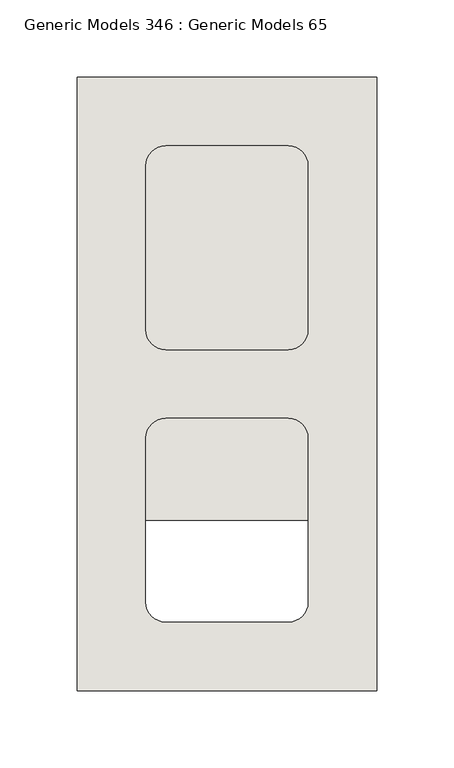
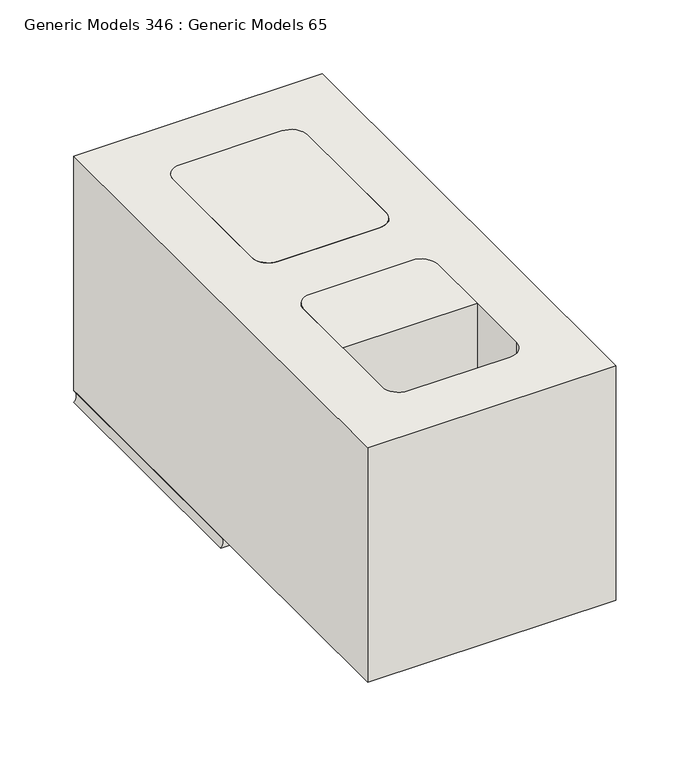
"""IFC4 building model written with IfcOpenShell, lengths in millimetres: wall geometry, Generic Models 346 : Generic Models 65."""

from ifc_helpers import new_model, si_unit, point, frame, frame_2d, origin, place, context, project, spatial, polyline, circle_curve, trimmed, segment, composite_curve, outline, extrude, source, transform, mapped, element, save
from ifc_brep_helpers import plane_surface, revolved_surface, advanced_brep


def generic_models_346_generic_models_65_9e6e97e0(model_context):
    return source(origin(), model_context, "Body", "SolidModel", [
        advanced_brep(
        [(430198.2125, 503.2375, 619.125), (430004.5375, 503.2375, 619.125), (430004.5375, 503.2375, 609.6), (430198.2125, 503.2375, 609.6), (430198.2125, 701.675, 619.125), (430198.2125, 701.675, 609.6), (430004.5375, 701.675, 609.6), (430004.5375, 701.675, 619.125), (430153.7625, 538.1625, 619.125), (430141.0625, 525.4625, 619.125), (430061.6875, 525.4625, 619.125), (430048.9875, 538.1625, 619.125), (430048.9875, 644.525, 619.125), (430061.6875, 657.225, 619.125), (430141.0625, 657.225, 619.125), (430153.7625, 644.525, 619.125), (430141.0625, 525.4625, 609.6), (430153.7625, 538.1625, 609.6), (430061.6875, 525.4625, 609.6), (430048.9875, 538.1625, 609.6), (430048.9875, 644.525, 609.6), (430061.6875, 657.225, 609.6), (430141.0625, 657.225, 609.6), (430153.7625, 644.525, 609.6)],
        [
            (0, 1),
            (1, 2, circle_curve(frame((429999.6545028, 503.2375, 614.3625), z_axis=(0.0, 1.0, 0.0), x_axis=(1.0, 0.0, 0.0)), 6.8209287)),
            (2, 3),
            (3, 0, circle_curve(frame((430203.0954972, 503.2375, 614.3625), z_axis=(0.0, 1.0, 0.0), x_axis=(-1.0, 0.0, 0.0)), 6.8209287)),
            (4, 5, circle_curve(frame((430203.0954972, 701.675, 614.3625), z_axis=(0.0, -1.0, 0.0), x_axis=(-1.0, 0.0, 0.0)), 6.8209287)),
            (5, 6),
            (6, 7, circle_curve(frame((429999.6545028, 701.675, 614.3625), z_axis=(0.0, -1.0, 0.0), x_axis=(1.0, 0.0, 0.0)), 6.8209287)),
            (7, 4),
            (0, 4),
            (7, 1),
            (8, 9, circle_curve(frame((430141.0625, 538.1625, 619.125), z_axis=(0.0, 0.0, -1.0), x_axis=(-1.0, 0.0, 0.0)), 12.7)),
            (9, 10),
            (10, 11, circle_curve(frame((430061.6875, 538.1625, 619.125), z_axis=(0.0, 0.0, -1.0), x_axis=(-1.0, 0.0, 0.0)), 12.7)),
            (11, 12),
            (12, 13, circle_curve(frame((430061.6875, 644.525, 619.125), z_axis=(0.0, 0.0, -1.0), x_axis=(-1.0, 0.0, 0.0)), 12.7)),
            (13, 14),
            (14, 15, circle_curve(frame((430141.0625, 644.525, 619.125), z_axis=(0.0, 0.0, -1.0), x_axis=(-1.0, 0.0, 0.0)), 12.7)),
            (15, 8),
            (16, 9),
            (8, 17),
            (17, 16, circle_curve(frame((430141.0625, 538.1625, 609.6), z_axis=(0.0, 0.0, -1.0), x_axis=(-1.0, 0.0, 0.0)), 12.7)),
            (16, 18),
            (18, 10),
            (18, 19, circle_curve(frame((430061.6875, 538.1625, 609.6), z_axis=(0.0, 0.0, -1.0), x_axis=(-1.0, 0.0, 0.0)), 12.7)),
            (19, 11),
            (19, 20),
            (20, 12),
            (20, 21, circle_curve(frame((430061.6875, 644.525, 609.6), z_axis=(0.0, 0.0, -1.0), x_axis=(-1.0, 0.0, 0.0)), 12.7)),
            (21, 13),
            (21, 22),
            (22, 14),
            (22, 23, circle_curve(frame((430141.0625, 644.525, 609.6), z_axis=(0.0, 0.0, -1.0), x_axis=(-1.0, 0.0, 0.0)), 12.7)),
            (23, 15),
            (23, 17),
            (6, 2),
            (5, 3),
        ],
        [
            plane_surface(frame((430101.375, 503.2375, 619.521875), z_axis=(0.0, -1.0, 0.0), x_axis=(0.0, 0.0, 1.0))),
            plane_surface(frame((430101.375, 701.675, 619.521875), z_axis=(0.0, 1.0, 0.0), x_axis=(0.0, 0.0, 1.0))),
            plane_surface(frame((430198.2125, 503.2375, 619.125), z_axis=(0.0, 0.0, 1.0), x_axis=(0.0, 1.0, 0.0))),
            revolved_surface(polyline([(430128.3625, 538.1625, 619.125), (430128.3625, 538.1625, 609.6)]), (430141.0625, 538.1625, 803.275), (0.0, 0.0, 1.0)),
            plane_surface(frame((430061.6875, 525.4625, 803.275), z_axis=(0.0, 1.0, 0.0), x_axis=(0.0, 0.0, -1.0))),
            revolved_surface(polyline([(430048.9875, 538.1625, 619.125), (430048.9875, 538.1625, 609.6)]), (430061.6875, 538.1625, 803.275), (0.0, 0.0, 1.0)),
            plane_surface(frame((430048.9875, 644.525, 803.275), z_axis=(1.0, 0.0, 0.0), x_axis=(0.0, 0.0, -1.0))),
            revolved_surface(polyline([(430048.9875, 644.525, 619.125), (430048.9875, 644.525, 609.6)]), (430061.6875, 644.525, 803.275), (0.0, 0.0, 1.0)),
            plane_surface(frame((430141.0625, 657.225, 803.275), z_axis=(0.0, -1.0, 0.0), x_axis=(0.0, 0.0, -1.0))),
            revolved_surface(polyline([(430128.3625, 644.525, 619.125), (430128.3625, 644.525, 609.6)]), (430141.0625, 644.525, 803.275), (0.0, 0.0, 1.0)),
            plane_surface(frame((430153.7625, 538.1625, 803.275), z_axis=(-1.0, 0.0, 0.0), x_axis=(0.0, 0.0, -1.0))),
            revolved_surface(polyline([(430006.4754315, 701.675, 614.3625), (430006.4754315, 503.2375, 614.3625)]), (429999.6545028, 503.2375, 614.3625), (0.0, 1.0, 0.0)),
            plane_surface(frame((430004.5375, 503.2375, 609.6), z_axis=(0.0, 0.0, -1.0), x_axis=(0.0, 1.0, 0.0))),
            revolved_surface(polyline([(430196.2745685, 701.675, 614.3625), (430196.2745685, 503.2375, 614.3625)]), (430203.0954972, 503.2375, 614.3625), (0.0, 1.0, 0.0)),
        ],
        [
            (0, [[1, 2, 3, 4]]),
            (1, [[5, 6, 7, 8]]),
            (2, [[-1, 9, -8, 10], [11, 12, 13, 14, 15, 16, 17, 18]]),
            (3, [[19, -11, 20, 21]]),
            (4, [[-19, 22, 23, -12]]),
            (5, [[-23, 24, 25, -13]]),
            (6, [[-25, 26, 27, -14]]),
            (7, [[-27, 28, 29, -15]]),
            (8, [[-29, 30, 31, -16]]),
            (9, [[-31, 32, 33, -17]]),
            (10, [[-33, 34, -20, -18]]),
            (11, [[-2, -10, -7, 35]]),
            (12, [[-3, -35, -6, 36], [-21, -34, -32, -30, -28, -26, -24, -22]]),
            (13, [[-4, -36, -5, -9]]),
        ],
    ),
        extrude(outline(composite_curve([segment(trimmed(circle_curve(frame_2d((430141.0625, 538.1625)), 12.7), [point((430153.7625, 538.1625))], [point((430141.0625, 525.4625))], False, "CARTESIAN"), True, "CONTINUOUS"), segment(polyline([(430141.0625, 525.4625), (430061.6875, 525.4625)]), True, "CONTINUOUS"), segment(trimmed(circle_curve(frame_2d((430061.6875, 538.1625)), 12.7), [point((430061.6875, 525.4625))], [point((430048.9875, 538.1625))], False, "CARTESIAN"), True, "CONTINUOUS"), segment(polyline([(430048.9875, 538.1625), (430048.9875, 644.525)]), True, "CONTINUOUS"), segment(trimmed(circle_curve(frame_2d((430061.6875, 644.525)), 12.7), [point((430048.9875, 644.525))], [point((430061.6875, 657.225))], False, "CARTESIAN"), True, "CONTINUOUS"), segment(polyline([(430061.6875, 657.225), (430141.0625, 657.225)]), True, "CONTINUOUS"), segment(trimmed(circle_curve(frame_2d((430141.0625, 644.525)), 12.7), [point((430141.0625, 657.225))], [point((430153.7625, 644.525))], False, "CARTESIAN"), True, "CONTINUOUS"), segment(polyline([(430153.7625, 644.525), (430153.7625, 538.1625)]), True, "CONTINUOUS")], self_intersect=False)), frame((0.0, 0.0, 609.6), z_axis=(0.0, 0.0, 1.0), x_axis=(1.0, 0.0, 0.0)), (0.0, 0.0, 1.0), 203.2),
        extrude(outline(composite_curve([segment(trimmed(circle_curve(frame_2d((430061.6875, 468.3125)), 12.7), [point((430048.9875, 468.3125))], [point((430061.6875, 481.0125))], False, "CARTESIAN"), True, "CONTINUOUS"), segment(polyline([(430061.6875, 481.0125), (430141.0625, 481.0125)]), True, "CONTINUOUS"), segment(trimmed(circle_curve(frame_2d((430141.0625, 468.3125)), 12.7), [point((430141.0625, 481.0125))], [point((430153.7625, 468.3125))], False, "CARTESIAN"), True, "CONTINUOUS"), segment(polyline([(430153.7625, 468.3125), (430153.7625, 415.13125), (430048.9875, 415.13125), (430048.9875, 468.3125)]), True, "CONTINUOUS")], self_intersect=False)), frame((0.0, 0.0, 609.6), z_axis=(0.0, 0.0, 1.0), x_axis=(1.0, 0.0, 0.0)), (0.0, 0.0, 1.0), 203.2),
        extrude(outline(polyline([(430198.2125, 304.8), (430004.5375, 304.8), (430004.5375, 701.675), (430198.2125, 701.675), (430198.2125, 304.8)]), holes=[composite_curve([segment(polyline([(430153.7625, 538.1625), (430153.7625, 644.525)]), True, "CONTINUOUS"), segment(trimmed(circle_curve(frame_2d((430141.0625, 644.525)), 12.7), [point((430153.7625, 644.525))], [point((430141.0625, 657.225))], True, "CARTESIAN"), True, "CONTINUOUS"), segment(polyline([(430141.0625, 657.225), (430061.6875, 657.225)]), True, "CONTINUOUS"), segment(trimmed(circle_curve(frame_2d((430061.6875, 644.525)), 12.7), [point((430061.6875, 657.225))], [point((430048.9875, 644.525))], True, "CARTESIAN"), True, "CONTINUOUS"), segment(polyline([(430048.9875, 644.525), (430048.9875, 538.1625)]), True, "CONTINUOUS"), segment(trimmed(circle_curve(frame_2d((430061.6875, 538.1625)), 12.7), [point((430048.9875, 538.1625))], [point((430061.6875, 525.4625))], True, "CARTESIAN"), True, "CONTINUOUS"), segment(polyline([(430061.6875, 525.4625), (430141.0625, 525.4625)]), True, "CONTINUOUS"), segment(trimmed(circle_curve(frame_2d((430141.0625, 538.1625)), 12.7), [point((430141.0625, 525.4625))], [point((430153.7625, 538.1625))], True, "CARTESIAN"), True, "CONTINUOUS")], self_intersect=False), composite_curve([segment(polyline([(430048.9875, 468.3125), (430048.9875, 361.95)]), True, "CONTINUOUS"), segment(trimmed(circle_curve(frame_2d((430061.6875, 361.95)), 12.7), [point((430048.9875, 361.95))], [point((430061.6875, 349.25))], True, "CARTESIAN"), True, "CONTINUOUS"), segment(polyline([(430061.6875, 349.25), (430141.0625, 349.25)]), True, "CONTINUOUS"), segment(trimmed(circle_curve(frame_2d((430141.0625, 361.95)), 12.7), [point((430141.0625, 349.25))], [point((430153.7625, 361.95))], True, "CARTESIAN"), True, "CONTINUOUS"), segment(polyline([(430153.7625, 361.95), (430153.7625, 468.3125)]), True, "CONTINUOUS"), segment(trimmed(circle_curve(frame_2d((430141.0625, 468.3125)), 12.7), [point((430153.7625, 468.3125))], [point((430141.0625, 481.0125))], True, "CARTESIAN"), True, "CONTINUOUS"), segment(polyline([(430141.0625, 481.0125), (430061.6875, 481.0125)]), True, "CONTINUOUS"), segment(trimmed(circle_curve(frame_2d((430061.6875, 468.3125)), 12.7), [point((430061.6875, 481.0125))], [point((430048.9875, 468.3125))], True, "CARTESIAN"), True, "CONTINUOUS")], self_intersect=False)]), frame((0.0, 0.0, 619.125), z_axis=(0.0, 0.0, 1.0), x_axis=(1.0, 0.0, 0.0)), (0.0, 0.0, 1.0), 193.675),
    ])


if __name__ == "__main__":
    model = new_model("IFC4")
    model_context = context("Model", 3, world=origin())
    ifc_project = project(units=[si_unit("LENGTHUNIT", "METRE", prefix="MILLI")], contexts=[model_context])
    site = spatial("IfcSite", under=ifc_project)
    building = spatial("IfcBuilding", under=site)
    placement = place(None, origin())
    generic_models_346_generic_models_65_shape = generic_models_346_generic_models_65_9e6e97e0(model_context)
    element("IfcWall", 1, ObjectType="Generic Models 346 : Generic Models 65", at=placement, inside=building, context=model_context, shape_type="MappedRepresentation", body=[
        mapped(generic_models_346_generic_models_65_shape, transform((0.0, 0.0, 0.0), x_axis=(1.0, 0.0, 0.0), y_axis=(0.0, 1.0, 0.0), z_axis=(0.0, 0.0, 1.0))),
    ])
    save(model, "model.ifc")

# Revit data of these elements
# Element 1 (IfcWall, "Generic Models 346 : Generic Models 65")
#   Materials on its faces: "CMU (SEE 'WALL TAG' FOR SIZE)", "FILL CORE IF APPLICABLE - SEE STRUCTURAL DWGS FOR DETAILS", "MORTAR JOINT"
# Materials
#   "CMU (SEE 'WALL TAG' FOR SIZE)": class "Masonry", colour RGB 203 203 199, transparency 0, Description = "Concrete masonry units", Cost = 0
#   "FILL CORE IF APPLICABLE - SEE STRUCTURAL DWGS FOR DETAILS": class "Generic", colour RGB 170 170 170, transparency 0, Cost = 0
#   "MORTAR JOINT": class "Generic", colour RGB 120 120 120, transparency 0, Cost = 0
